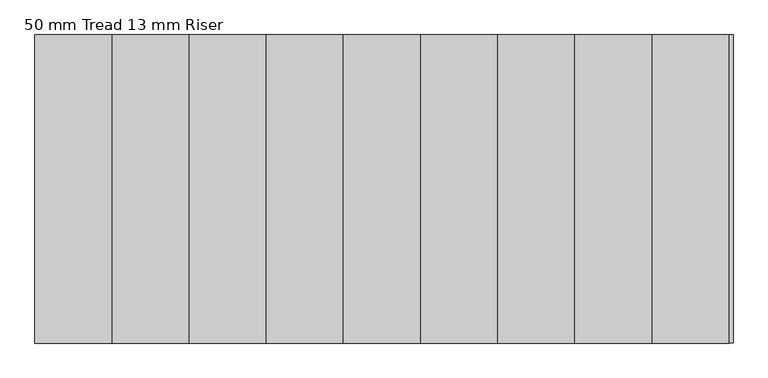
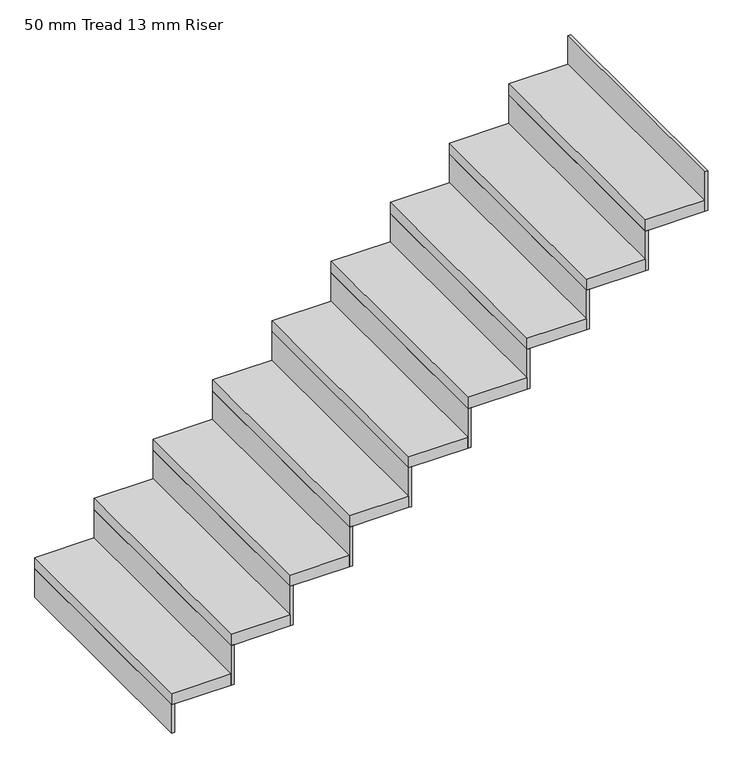
"""IFC4 building model written with IfcOpenShell, lengths in millimetres: stair flight geometry, 50 mm Tread 13 mm Riser."""

from ifc_helpers import new_model, si_unit, frame, origin, origin_with_axes, place, context, project, spatial, polyline, outline, extrude, source, transform, mapped, element, save


def stair_flight_50_mm_tread_13_mm_riser_f9bf53a1(model_context):
    return source(origin(), model_context, "Body", "SweptSolid", [
        extrude(outline(polyline([(28075.5737371, -1705.6098174), (28063.0737371, -1705.6098174), (28063.0737371, -705.6098174), (28075.5737371, -705.6098174), (28075.5737371, -1705.6098174)])), origin_with_axes(), (0.0, 0.0, 1.0), 126.4705882),
        extrude(outline(polyline([(28313.0737371, -705.6098174), (28313.0737371, -1705.6098174), (28063.0737371, -1705.6098174), (28063.0737371, -705.6098174), (28313.0737371, -705.6098174)])), frame((0.0, 0.0, 126.4705882), z_axis=(0.0, 0.0, 1.0), x_axis=(1.0, 0.0, 0.0)), (0.0, 0.0, 1.0), 50.0),
        extrude(outline(polyline([(28325.5737371, -1705.6098174), (28313.0737371, -1705.6098174), (28313.0737371, -705.6098174), (28325.5737371, -705.6098174), (28325.5737371, -1705.6098174)])), frame((0.0, 0.0, 126.4705882), z_axis=(0.0, 0.0, 1.0), x_axis=(1.0, 0.0, 0.0)), (0.0, 0.0, 1.0), 176.4705882),
        extrude(outline(polyline([(28563.0737371, -705.6098174), (28563.0737371, -1705.6098174), (28313.0737371, -1705.6098174), (28313.0737371, -705.6098174), (28563.0737371, -705.6098174)])), frame((0.0, 0.0, 302.9411765), z_axis=(0.0, 0.0, 1.0), x_axis=(1.0, 0.0, 0.0)), (0.0, 0.0, 1.0), 50.0),
        extrude(outline(polyline([(28575.5737371, -1705.6098174), (28563.0737371, -1705.6098174), (28563.0737371, -705.6098174), (28575.5737371, -705.6098174), (28575.5737371, -1705.6098174)])), frame((0.0, 0.0, 302.9411765), z_axis=(0.0, 0.0, 1.0), x_axis=(1.0, 0.0, 0.0)), (0.0, 0.0, 1.0), 176.4705882),
        extrude(outline(polyline([(28813.0737371, -705.6098174), (28813.0737371, -1705.6098174), (28563.0737371, -1705.6098174), (28563.0737371, -705.6098174), (28813.0737371, -705.6098174)])), frame((0.0, 0.0, 479.4117647), z_axis=(0.0, 0.0, 1.0), x_axis=(1.0, 0.0, 0.0)), (0.0, 0.0, 1.0), 50.0),
        extrude(outline(polyline([(28825.5737371, -1705.6098174), (28813.0737371, -1705.6098174), (28813.0737371, -705.6098174), (28825.5737371, -705.6098174), (28825.5737371, -1705.6098174)])), frame((0.0, 0.0, 479.4117647), z_axis=(0.0, 0.0, 1.0), x_axis=(1.0, 0.0, 0.0)), (0.0, 0.0, 1.0), 176.4705882),
        extrude(outline(polyline([(29063.0737371, -705.6098174), (29063.0737371, -1705.6098174), (28813.0737371, -1705.6098174), (28813.0737371, -705.6098174), (29063.0737371, -705.6098174)])), frame((0.0, 0.0, 655.8823529), z_axis=(0.0, 0.0, 1.0), x_axis=(1.0, 0.0, 0.0)), (0.0, 0.0, 1.0), 50.0),
        extrude(outline(polyline([(29075.5737371, -1705.6098174), (29063.0737371, -1705.6098174), (29063.0737371, -705.6098174), (29075.5737371, -705.6098174), (29075.5737371, -1705.6098174)])), frame((0.0, 0.0, 655.8823529), z_axis=(0.0, 0.0, 1.0), x_axis=(1.0, 0.0, 0.0)), (0.0, 0.0, 1.0), 176.4705882),
        extrude(outline(polyline([(29313.0737371, -705.6098174), (29313.0737371, -1705.6098174), (29063.0737371, -1705.6098174), (29063.0737371, -705.6098174), (29313.0737371, -705.6098174)])), frame((0.0, 0.0, 832.3529412), z_axis=(0.0, 0.0, 1.0), x_axis=(1.0, 0.0, 0.0)), (0.0, 0.0, 1.0), 50.0),
        extrude(outline(polyline([(29325.5737371, -1705.6098174), (29313.0737371, -1705.6098174), (29313.0737371, -705.6098174), (29325.5737371, -705.6098174), (29325.5737371, -1705.6098174)])), frame((0.0, 0.0, 832.3529412), z_axis=(0.0, 0.0, 1.0), x_axis=(1.0, 0.0, 0.0)), (0.0, 0.0, 1.0), 176.4705882),
        extrude(outline(polyline([(29563.0737371, -705.6098174), (29563.0737371, -1705.6098174), (29313.0737371, -1705.6098174), (29313.0737371, -705.6098174), (29563.0737371, -705.6098174)])), frame((0.0, 0.0, 1008.8235294), z_axis=(0.0, 0.0, 1.0), x_axis=(1.0, 0.0, 0.0)), (0.0, 0.0, 1.0), 50.0),
        extrude(outline(polyline([(29575.5737371, -1705.6098174), (29563.0737371, -1705.6098174), (29563.0737371, -705.6098174), (29575.5737371, -705.6098174), (29575.5737371, -1705.6098174)])), frame((0.0, 0.0, 1008.8235294), z_axis=(0.0, 0.0, 1.0), x_axis=(1.0, 0.0, 0.0)), (0.0, 0.0, 1.0), 176.4705882),
        extrude(outline(polyline([(29813.0737371, -705.6098174), (29813.0737371, -1705.6098174), (29563.0737371, -1705.6098174), (29563.0737371, -705.6098174), (29813.0737371, -705.6098174)])), frame((0.0, 0.0, 1185.2941176), z_axis=(0.0, 0.0, 1.0), x_axis=(1.0, 0.0, 0.0)), (0.0, 0.0, 1.0), 50.0),
        extrude(outline(polyline([(29825.5737371, -1705.6098174), (29813.0737371, -1705.6098174), (29813.0737371, -705.6098174), (29825.5737371, -705.6098174), (29825.5737371, -1705.6098174)])), frame((0.0, 0.0, 1185.2941176), z_axis=(0.0, 0.0, 1.0), x_axis=(1.0, 0.0, 0.0)), (0.0, 0.0, 1.0), 176.4705882),
        extrude(outline(polyline([(30063.0737371, -705.6098174), (30063.0737371, -1705.6098174), (29813.0737371, -1705.6098174), (29813.0737371, -705.6098174), (30063.0737371, -705.6098174)])), frame((0.0, 0.0, 1361.7647059), z_axis=(0.0, 0.0, 1.0), x_axis=(1.0, 0.0, 0.0)), (0.0, 0.0, 1.0), 50.0),
        extrude(outline(polyline([(30075.5737371, -1705.6098174), (30063.0737371, -1705.6098174), (30063.0737371, -705.6098174), (30075.5737371, -705.6098174), (30075.5737371, -1705.6098174)])), frame((0.0, 0.0, 1361.7647059), z_axis=(0.0, 0.0, 1.0), x_axis=(1.0, 0.0, 0.0)), (0.0, 0.0, 1.0), 176.4705882),
        extrude(outline(polyline([(30325.5737371, -1705.6098174), (30313.0737371, -1705.6098174), (30313.0737371, -705.6098174), (30325.5737371, -705.6098174), (30325.5737371, -1705.6098174)])), frame((0.0, 0.0, 1538.2352941), z_axis=(0.0, 0.0, 1.0), x_axis=(1.0, 0.0, 0.0)), (0.0, 0.0, 1.0), 176.4705882),
        extrude(outline(polyline([(30313.0737371, -705.6098174), (30313.0737371, -1705.6098174), (30063.0737371, -1705.6098174), (30063.0737371, -705.6098174), (30313.0737371, -705.6098174)])), frame((0.0, 0.0, 1538.2352941), z_axis=(0.0, 0.0, 1.0), x_axis=(1.0, 0.0, 0.0)), (0.0, 0.0, 1.0), 50.0),
    ])


if __name__ == "__main__":
    model = new_model("IFC4")
    model_context = context("Model", 3, world=origin())
    ifc_project = project(units=[si_unit("LENGTHUNIT", "METRE", prefix="MILLI")], contexts=[model_context])
    site = spatial("IfcSite", under=ifc_project)
    building = spatial("IfcBuilding", under=site)
    placement = place(None, origin())
    stair_flight_50_mm_tread_13_mm_riser_shape = stair_flight_50_mm_tread_13_mm_riser_f9bf53a1(model_context)
    element("IfcStairFlight", 1, ObjectType="50 mm Tread 13 mm Riser", at=placement, inside=building, context=model_context, shape_type="MappedRepresentation", body=[
        mapped(stair_flight_50_mm_tread_13_mm_riser_shape, transform((0.0, 0.0, 0.0), x_axis=(1.0, 0.0, 0.0), y_axis=(0.0, 1.0, 0.0), z_axis=(0.0, 0.0, 1.0))),
    ])
    save(model, "model.ifc")
